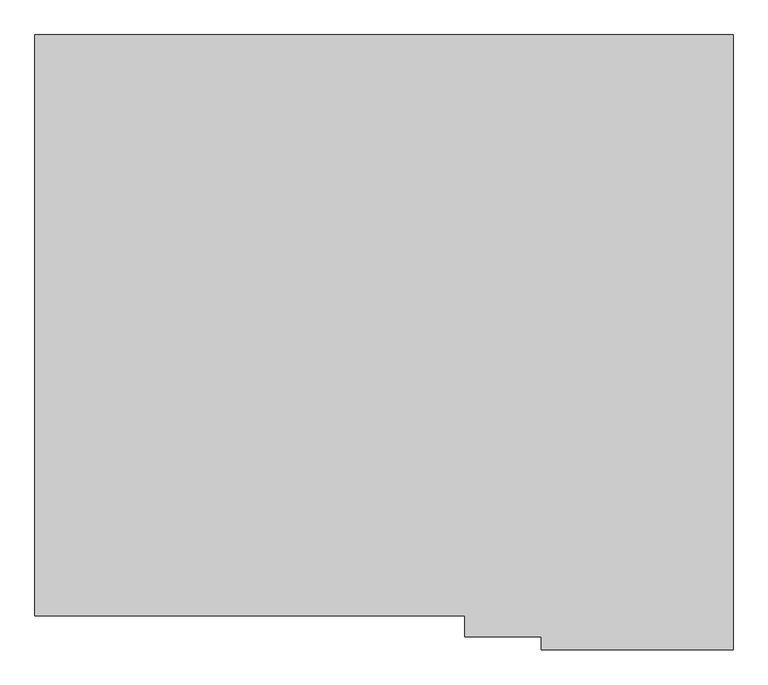
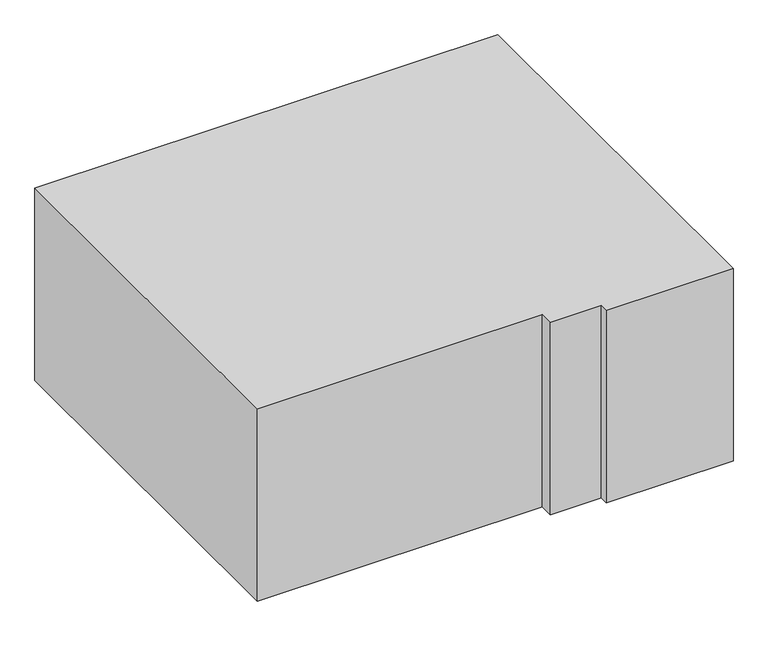
"""IFC4 building model written with IfcOpenShell, lengths in millimetres: proxy geometry, 0_3d."""

from ifc_helpers import new_model, si_unit, origin, origin_with_axes, place, context, project, spatial, polyline, outline, extrude, source, transform, mapped, element, save


def generic_models_a5f5eca8(model_context):
    return source(origin(), model_context, "Body", "SweptSolid", [
        extrude(outline(polyline([(6547.9290232, 5772.0), (6547.9290232, 0.0), (4750.0, 0.0), (4750.0, 122.0), (4031.4631733, 122.0), (4031.4631733, 322.0), (0.0, 322.0), (0.0, 5772.0), (6547.9290232, 5772.0)])), origin_with_axes(), (0.0, 0.0, 1.0), 2880.0),
    ])


if __name__ == "__main__":
    model = new_model("IFC4")
    model_context = context("Model", 3, world=origin())
    ifc_project = project(units=[si_unit("LENGTHUNIT", "METRE", prefix="MILLI")], contexts=[model_context])
    site = spatial("IfcSite", under=ifc_project)
    building = spatial("IfcBuilding", under=site)
    placement = place(None, origin())
    generic_models_shape = generic_models_a5f5eca8(model_context)
    element("IfcBuildingElementProxy", 1, Name="0_3d", ObjectType="0_3d", at=placement, inside=building, context=model_context, shape_type="MappedRepresentation", body=[
        mapped(generic_models_shape, transform((0.0, 0.0, 0.0), x_axis=(1.0, 0.0, 0.0), y_axis=(0.0, 1.0, 0.0), z_axis=(0.0, 0.0, 1.0))),
    ])
    save(model, "model.ifc")

# Revit data of these elements
# Element 1 (IfcBuildingElementProxy, "0_3d")
#   Materials on its faces: "*1"
# Materials
#   "*1": class "Unassigned", colour RGB 175 175 175, transparency 0
